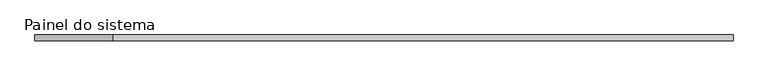
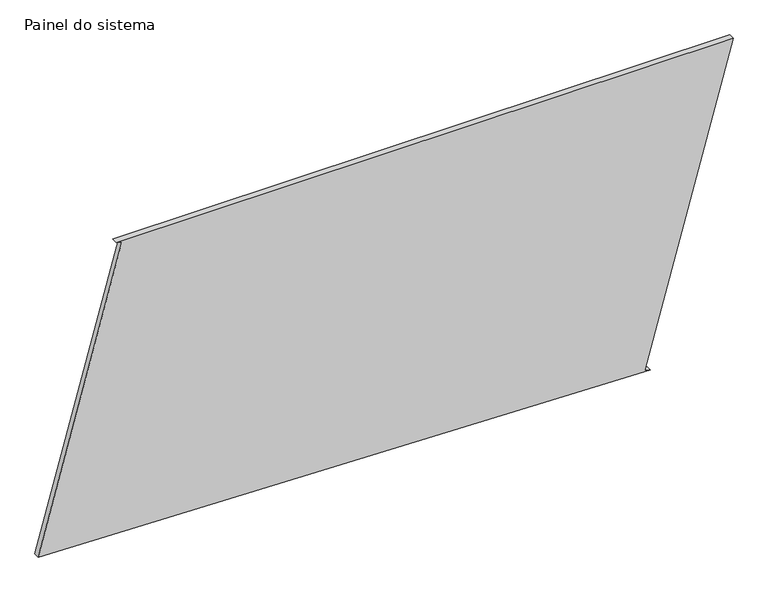
"""IFC4 building model written with IfcOpenShell, lengths in millimetres: plate geometry, Painel do sistema : Envidraçado."""

from ifc_helpers import new_model, si_unit, frame, origin, place, context, project, spatial, polyline, outline, extrude, source, transform, mapped, element, save


def painel_do_sistema_340d9e0c(model_context):
    return source(origin(), model_context, "Body", "SweptSolid", [
        extrude(outline(polyline([(0.0, 1134.4287763), (6.6310485, 1110.3242291), (1380.6696296, 1488.3158366), (1380.6696296, -1153.9542279), (1374.0385811, -1129.8496807), (70.9770358, -1488.3158366), (0.0, 1134.4287763)])), frame((0.0, 24.5, 0.0), z_axis=(0.0, 1.0, 0.0), x_axis=(0.0, 0.0, 1.0)), (0.0, 0.0, 1.0), 25.0),
    ])


if __name__ == "__main__":
    model = new_model("IFC4")
    model_context = context("Model", 3, world=origin())
    ifc_project = project(units=[si_unit("LENGTHUNIT", "METRE", prefix="MILLI")], contexts=[model_context])
    site = spatial("IfcSite", under=ifc_project)
    building = spatial("IfcBuilding", under=site)
    placement = place(None, origin())
    painel_do_sistema_shape = painel_do_sistema_340d9e0c(model_context)
    element("IfcPlate", 1, ObjectType="Painel do sistema : Envidraçado", at=placement, inside=building, context=model_context, shape_type="MappedRepresentation", body=[
        mapped(painel_do_sistema_shape, transform((0.0, 0.0, 0.0), x_axis=(1.0, 0.0, 0.0), y_axis=(0.0, 1.0, 0.0), z_axis=(0.0, 0.0, 1.0))),
    ])
    save(model, "model.ifc")

# Revit data of these elements
# Type "Painel do sistema : Envidraçado"
#   Construction Type Id = "GSP4R"
#   Analytic Construction = "Vidraça única Pilkington 1/8 pol"
#   Visual Light Transmittance = 0.9
#   Solar Heat Gain Coefficient = 0.86
#   Heat Transfer Coefficient (U) = 6.7069 W/(m²·K)
# Element 1 (IfcPlate, "Painel do sistema : Envidraçado")
#   Materials on its faces: "Vidro"
# Materials
#   "Vidro": class "Vidro", colour RGB 0 128 192, transparency 0.9, Description = "Vidro de sílica", Cost = 0
